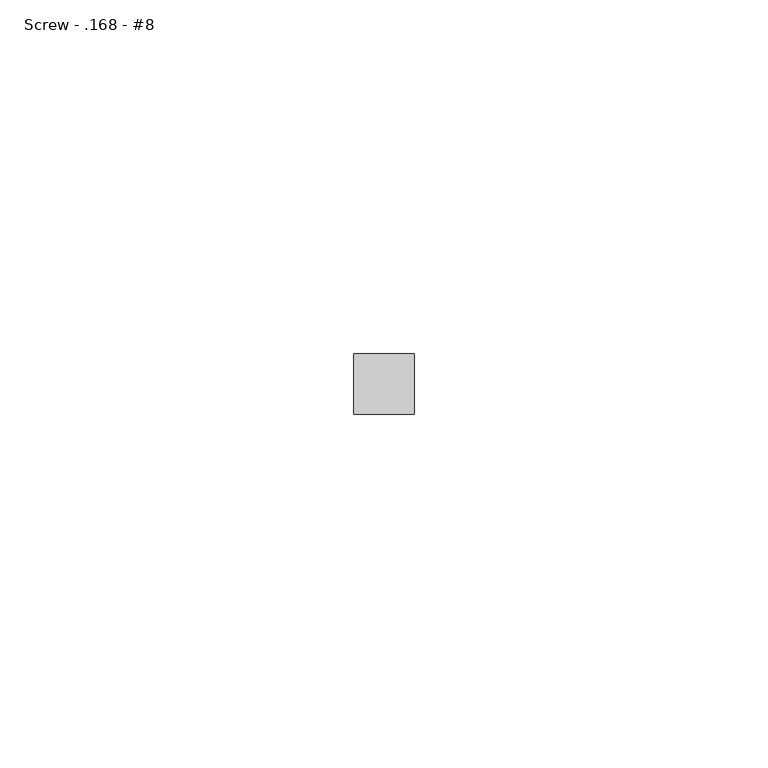
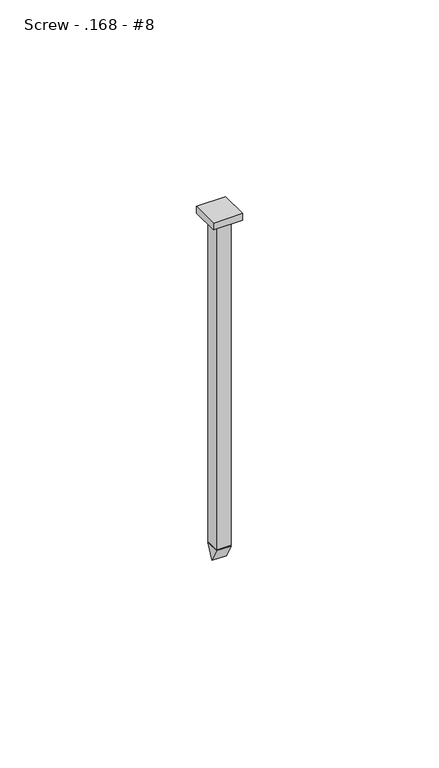
"""IFC4 building model written with IfcOpenShell, lengths in millimetres: fastener geometry, 060523 - W_P_C - Fastenings - Generic - SQUARE : Screw - .168 - #8."""

from ifc_helpers import new_model, si_unit, frame, origin, origin_with_axes, place, context, project, spatial, polyline, outline, extrude, source, transform, mapped, element, save


def screw_168_8_1d1329a1(model_context):
    return source(origin(), model_context, "Body", "SweptSolid", [
        extrude(outline(polyline([(0.0, -105.8672), (-2.1336, -101.6), (2.1336, -101.6), (0.0, -105.8672)])), frame((-2.1336, 0.0, 0.0), z_axis=(1.0, 0.0, 0.0), x_axis=(0.0, 1.0, 0.0)), (0.0, 0.0, 1.0), 4.2672),
        extrude(outline(polyline([(-4.2672, -4.2672), (-4.2672, 4.2672), (4.2672, 4.2672), (4.2672, -4.2672), (-4.2672, -4.2672)])), origin_with_axes(), (0.0, 0.0, 1.0), 2.1336),
        extrude(outline(polyline([(-2.1336, 2.1336), (2.1336, 2.1336), (2.1336, -2.1336), (-2.1336, -2.1336), (-2.1336, 2.1336)])), frame((0.0, 0.0, -101.6), z_axis=(0.0, 0.0, 1.0), x_axis=(1.0, 0.0, 0.0)), (0.0, 0.0, 1.0), 101.6),
    ])


if __name__ == "__main__":
    model = new_model("IFC4")
    model_context = context("Model", 3, world=origin())
    ifc_project = project(units=[si_unit("LENGTHUNIT", "METRE", prefix="MILLI")], contexts=[model_context])
    site = spatial("IfcSite", under=ifc_project)
    building = spatial("IfcBuilding", under=site)
    placement = place(None, origin())
    screw_168_8_shape = screw_168_8_1d1329a1(model_context)
    element("IfcFastener", 1, ObjectType="060523 - W_P_C - Fastenings - Generic - SQUARE : Screw - .168 - #8", at=placement, inside=building, context=model_context, shape_type="MappedRepresentation", body=[
        mapped(screw_168_8_shape, transform((0.0, 0.0, 0.0), x_axis=(1.0, 0.0, 0.0), y_axis=(0.0, 1.0, 0.0), z_axis=(0.0, 0.0, 1.0))),
    ])
    save(model, "model.ifc")

# Revit data of these elements
# Type "060523 - W_P_C - Fastenings - Generic - SQUARE : Screw - .168 - #8"
#   Washer_Thickness = 0' - 0.00333"
#   Washer Radius = 0' - 0.094"
#   Washer Offset - Head = 0' - 0"
#   Washer Offset = 0' - 0"
#   Thickness_of_Substrate [instance default] = 0' - 1"
#   Side = 0' - 0 37/64"
#   Radius = 0' - 0.084"
#   Length [instance default] = 0' - 4"
#   Head Size = 0' - 1"
#   Head Radius = 0' - 0 1/2"
#   Head Height = 0' - 0.01"
#   Double Diameter = 0' - 0.336"
#   Diameter = 0' - 0.168"
#   Default Elevation = 4' - 0"
#   Washer_Nut_Visibility = no
#   Washer_Head_Visibility = no
#   Round_Head_Visibility = yes
#   Point Visibility = yes
#   Nut_Visibility = no
#   Hex_Head_Visiblilty = no
#   Washer Material = none
#   Bolt Material (Size) = AT SILL - FASTENER AT 24" O.C.
# Materials
#   "AT SILL - FASTENER AT 24\" O.C.": class "Generic", colour RGB 120 120 120, transparency 0, Cost = 0
